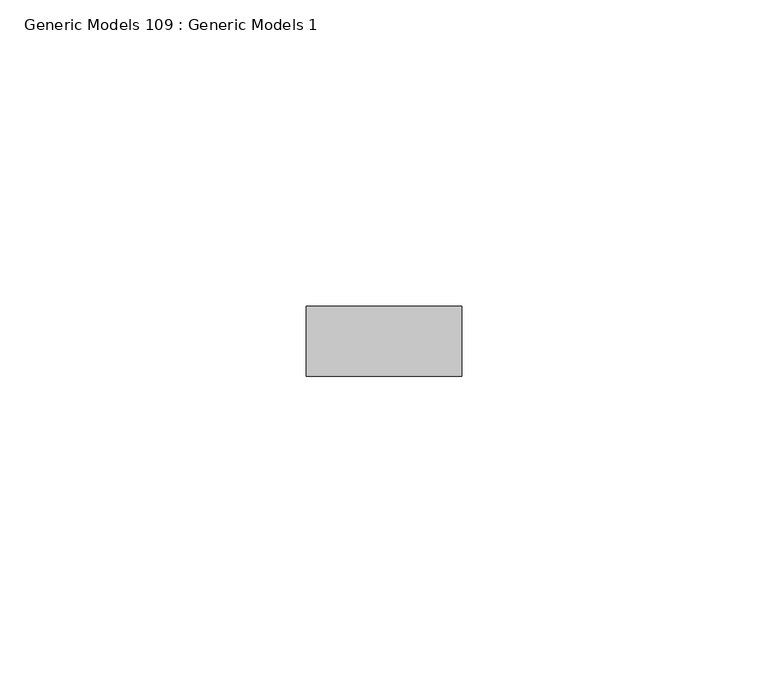
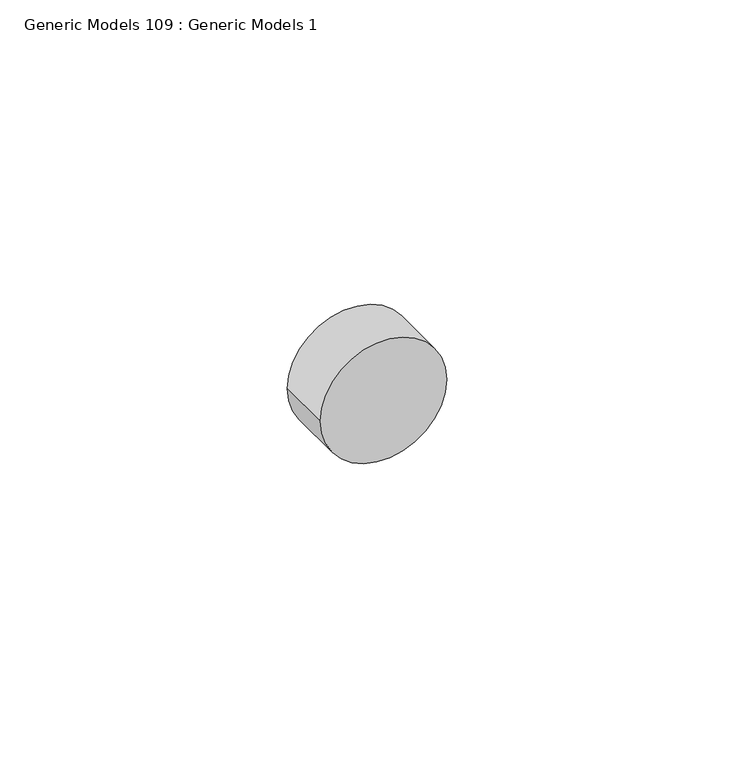
"""IFC4 building model written with IfcOpenShell, lengths in millimetres: proxy geometry, Generic Models 109 : Generic Models 1."""

from ifc_helpers import new_model, si_unit, point, frame, frame_2d, origin, place, context, project, spatial, circle_curve, trimmed, segment, composite_curve, outline, extrude, source, transform, mapped, element, save


def generic_models_109_generic_models_1_f5edd009(model_context):
    return source(origin(), model_context, "Body", "SweptSolid", [
        extrude(outline(composite_curve([segment(trimmed(circle_curve(frame_2d((37688.9033735, 6569.3828124)), 12.7), [point((37688.9033735, 6556.6828124))], [point((37688.9033735, 6582.0828124))], False, "CARTESIAN"), True, "CONTINUOUS"), segment(trimmed(circle_curve(frame_2d((37688.9033735, 6569.3828124)), 12.7), [point((37688.9033735, 6582.0828124))], [point((37688.9033735, 6556.6828124))], False, "CARTESIAN"), True, "CONTINUOUS")], self_intersect=False)), frame((0.0, 1836.9202358, 0.0), z_axis=(0.0, 1.0, 0.0), x_axis=(0.0, 0.0, 1.0)), (0.0, 0.0, 1.0), 11.4464372),
    ])


if __name__ == "__main__":
    model = new_model("IFC4")
    model_context = context("Model", 3, world=origin())
    ifc_project = project(units=[si_unit("LENGTHUNIT", "METRE", prefix="MILLI")], contexts=[model_context])
    site = spatial("IfcSite", under=ifc_project)
    building = spatial("IfcBuilding", under=site)
    placement = place(None, origin())
    generic_models_109_generic_models_1_shape = generic_models_109_generic_models_1_f5edd009(model_context)
    element("IfcBuildingElementProxy", 1, Name="Generic Models 109 : Generic Models 1", ObjectType="Generic Models 109 : Generic Models 1", at=placement, inside=building, context=model_context, shape_type="MappedRepresentation", body=[
        mapped(generic_models_109_generic_models_1_shape, transform((0.0, 0.0, 0.0), x_axis=(1.0, 0.0, 0.0), y_axis=(0.0, 1.0, 0.0), z_axis=(0.0, 0.0, 1.0))),
    ])
    save(model, "model.ifc")

# Revit data of these elements
# Element 1 (IfcBuildingElementProxy, "Generic Models 109 : Generic Models 1")
#   Materials on its faces: "S.S. LAG BOLT - SEE STRUCT. DWGS"
# Materials
#   "S.S. LAG BOLT - SEE STRUCT. DWGS": class "Generic", colour RGB 120 120 120, transparency 0, Cost = 0
